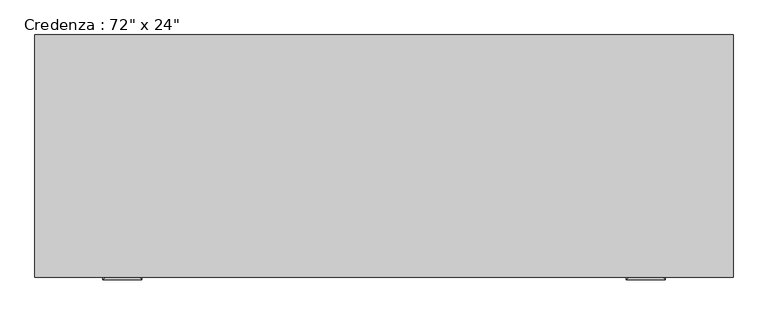
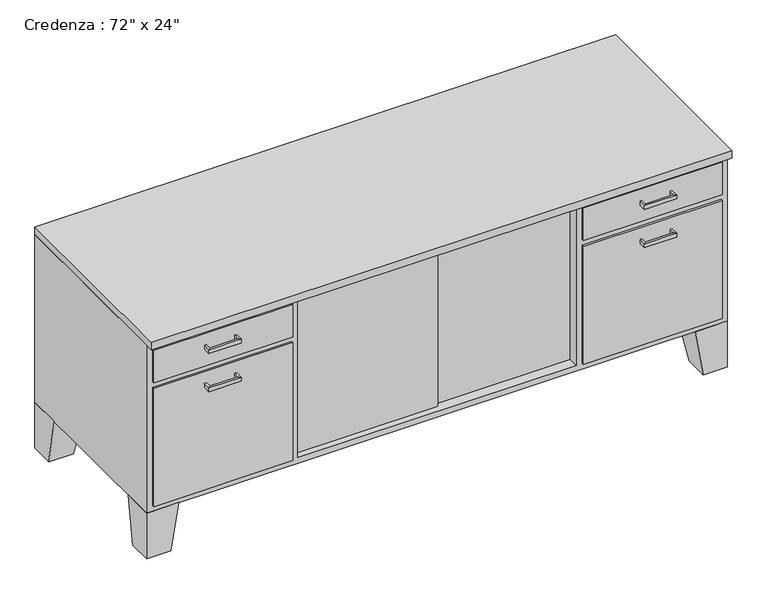
"""IFC4 building model written with IfcOpenShell, lengths in millimetres: furniture geometry."""

from ifc_helpers import new_model, si_unit, frame, origin, place, context, project, spatial, polyline, outline, extrude, faceted_brep, source, transform, mapped, element, save


def furniture_d4af3f8d(model_context):
    return source(origin(), model_context, "Body", "SolidModel", [
        extrude(outline(polyline([(531.7023176, -267.2714583), (46.8442623, -267.2714583), (46.8442623, -254.5714583), (531.7023176, -254.5714583), (531.7023176, -267.2714583)])), frame((0.0, 0.0, 171.45), z_axis=(0.0, 0.0, 1.0), x_axis=(1.0, 0.0, 0.0)), (0.0, 0.0, 1.0), 520.7),
        extrude(outline(polyline([(73.6254475, -279.9714583), (-378.6057377, -279.9714583), (-378.6057377, -267.2714583), (73.6254475, -267.2714583), (73.6254475, -279.9714583)])), frame((0.0, 0.0, 171.45), z_axis=(0.0, 0.0, 1.0), x_axis=(1.0, 0.0, 0.0)), (0.0, 0.0, 1.0), 520.7),
        faceted_brep([(872.3442623, 309.3803279, 152.4), (872.3442623, 207.7803279, 152.4), (973.9442623, 207.7803279, 152.4), (973.9442623, 309.3803279, 152.4), (897.7442623, 309.3803279, 0.0), (973.9442623, 309.3803279, 0.0), (973.9442623, 233.1803279, 0.0), (897.7442623, 233.1803279, 0.0)], [[[0, 1, 2, 3]], [[4, 5, 6, 7]], [[4, 7, 1, 0]], [[7, 6, 2, 1]], [[6, 5, 3, 2]], [[5, 4, 0, 3]]]),
        extrude(outline(polyline([(954.8942623, -306.5696721), (516.7442623, -306.5696721), (516.7442623, -300.2196721), (954.8942623, -300.2196721), (954.8942623, -306.5696721)])), frame((0.0, 0.0, 584.2), z_axis=(0.0, 0.0, 1.0), x_axis=(1.0, 0.0, 0.0)), (0.0, 0.0, 1.0), 107.95),
        extrude(outline(polyline([(954.8942623, -306.5696721), (516.7442623, -306.5696721), (516.7442623, -300.2196721), (954.8942623, -300.2196721), (954.8942623, -306.5696721)])), frame((0.0, 0.0, 171.45), z_axis=(0.0, 0.0, 1.0), x_axis=(1.0, 0.0, 0.0)), (0.0, 0.0, 1.0), 393.7),
        extrude(outline(polyline([(-397.6557377, -306.5696721), (-835.8057377, -306.5696721), (-835.8057377, -300.2196721), (-397.6557377, -300.2196721), (-397.6557377, -306.5696721)])), frame((0.0, 0.0, 584.2), z_axis=(0.0, 0.0, 1.0), x_axis=(1.0, 0.0, 0.0)), (0.0, 0.0, 1.0), 107.95),
        extrude(outline(polyline([(-397.6557377, -306.5696721), (-835.8057377, -306.5696721), (-835.8057377, -300.2196721), (-397.6557377, -300.2196721), (-397.6557377, -306.5696721)])), frame((0.0, 0.0, 171.45), z_axis=(0.0, 0.0, 1.0), x_axis=(1.0, 0.0, 0.0)), (0.0, 0.0, 1.0), 393.7),
        faceted_brep([(-753.2557377, -300.2196721, 152.4), (-753.2557377, -198.6196721, 152.4), (-854.8557377, -198.6196721, 152.4), (-854.8557377, -300.2196721, 152.4), (-778.6557377, -300.2196721, 0.0), (-854.8557377, -300.2196721, 0.0), (-854.8557377, -224.0196721, 0.0), (-778.6557377, -224.0196721, 0.0)], [[[0, 1, 2, 3]], [[4, 5, 6, 7]], [[4, 7, 1, 0]], [[7, 6, 2, 1]], [[6, 5, 3, 2]], [[5, 4, 0, 3]]]),
        faceted_brep([(-753.2557377, 309.3803279, 152.4), (-854.8557377, 309.3803279, 152.4), (-854.8557377, 207.7803279, 152.4), (-753.2557377, 207.7803279, 152.4), (-778.6557377, 309.3803279, 0.0), (-778.6557377, 233.1803279, 0.0), (-854.8557377, 233.1803279, 0.0), (-854.8557377, 309.3803279, 0.0)], [[[0, 1, 2, 3]], [[4, 5, 6, 7]], [[4, 7, 1, 0]], [[7, 6, 2, 1]], [[6, 5, 3, 2]], [[5, 4, 0, 3]]]),
        faceted_brep([(872.3442623, -300.2196721, 152.4), (973.9442623, -300.2196721, 152.4), (973.9442623, -198.6196721, 152.4), (872.3442623, -198.6196721, 152.4), (897.7442623, -300.2196721, 0.0), (897.7442623, -224.0196721, 0.0), (973.9442623, -224.0196721, 0.0), (973.9442623, -300.2196721, 0.0)], [[[0, 1, 2, 3]], [[4, 5, 6, 7]], [[4, 7, 1, 0]], [[7, 6, 2, 1]], [[6, 5, 3, 2]], [[5, 4, 0, 3]]]),
        faceted_brep([(973.9442623, 309.3803279, 711.2), (-854.8557377, 309.3803279, 711.2), (-854.8557377, -300.2196721, 711.2), (973.9442623, -300.2196721, 711.2), (973.9442623, 309.3803279, 152.4), (973.9442623, -300.2196721, 152.4), (-854.8557377, -300.2196721, 152.4), (-854.8557377, 309.3803279, 152.4), (-378.6057377, -300.2196721, 692.15), (497.6942623, -300.2196721, 692.15), (497.6942623, -300.2196721, 171.45), (-378.6057377, -300.2196721, 171.45), (497.6942623, 290.3303279, 692.15), (-378.6057377, 290.3303279, 692.15), (-378.6057377, 290.3303279, 171.45), (497.6942623, 290.3303279, 171.45)], [[[0, 1, 2, 3]], [[4, 5, 6, 7]], [[1, 0, 4, 7]], [[2, 1, 7, 6]], [[3, 2, 6, 5], [8, 9, 10, 11]], [[0, 3, 5, 4]], [[12, 13, 14, 15]], [[13, 12, 9, 8]], [[14, 13, 8, 11]], [[15, 14, 11, 10]], [[12, 15, 10, 9]]]),
        extrude(outline(polyline([(973.9442623, 309.3803279), (973.9442623, -325.6196721), (-854.8557377, -325.6196721), (-854.8557377, 309.3803279), (973.9442623, 309.3803279)])), frame((0.0, 0.0, 711.2), z_axis=(0.0, 0.0, 1.0), x_axis=(1.0, 0.0, 0.0)), (0.0, 0.0, 1.0), 25.4),
        faceted_brep([(-670.7057377, -306.5696721, 527.05), (-670.7057377, -306.5696721, 514.35), (-677.0557377, -306.5696721, 514.35), (-677.0557377, -306.5696721, 527.05), (-670.7057377, -325.6196721, 527.05), (-670.7057377, -325.6196721, 514.35), (-677.0557377, -331.9696721, 514.35), (-677.0557377, -331.9696721, 527.05), (-581.8057377, -325.6196721, 527.05), (-581.8057377, -325.6196721, 514.35), (-575.4557377, -331.9696721, 514.35), (-575.4557377, -331.9696721, 527.05), (-581.8057377, -306.5696721, 527.05), (-575.4557377, -306.5696721, 527.05), (-575.4557377, -306.5696721, 514.35), (-581.8057377, -306.5696721, 514.35)], [[[0, 1, 2, 3]], [[1, 0, 4, 5]], [[2, 1, 5, 6]], [[3, 2, 6, 7]], [[0, 3, 7, 4]], [[5, 4, 8, 9]], [[6, 5, 9, 10]], [[7, 6, 10, 11]], [[4, 7, 11, 8]], [[12, 13, 14, 15]], [[9, 8, 12, 15]], [[10, 9, 15, 14]], [[11, 10, 14, 13]], [[8, 11, 13, 12]]]),
        faceted_brep([(-670.7057377, -306.5696721, 654.05), (-670.7057377, -306.5696721, 641.35), (-677.0557377, -306.5696721, 641.35), (-677.0557377, -306.5696721, 654.05), (-670.7057377, -325.6196721, 654.05), (-670.7057377, -325.6196721, 641.35), (-677.0557377, -331.9696721, 641.35), (-677.0557377, -331.9696721, 654.05), (-581.8057377, -325.6196721, 654.05), (-581.8057377, -325.6196721, 641.35), (-575.4557377, -331.9696721, 641.35), (-575.4557377, -331.9696721, 654.05), (-581.8057377, -306.5696721, 654.05), (-575.4557377, -306.5696721, 654.05), (-575.4557377, -306.5696721, 641.35), (-581.8057377, -306.5696721, 641.35)], [[[0, 1, 2, 3]], [[1, 0, 4, 5]], [[2, 1, 5, 6]], [[3, 2, 6, 7]], [[0, 3, 7, 4]], [[5, 4, 8, 9]], [[6, 5, 9, 10]], [[7, 6, 10, 11]], [[4, 7, 11, 8]], [[12, 13, 14, 15]], [[9, 8, 12, 15]], [[10, 9, 15, 14]], [[11, 10, 14, 13]], [[8, 11, 13, 12]]]),
        faceted_brep([(700.8942623, -306.5696721, 654.1373112), (700.8942623, -306.5696721, 641.4373112), (694.5442623, -306.5696721, 641.4373112), (694.5442623, -306.5696721, 654.1373112), (700.8942623, -325.6196721, 654.1373112), (700.8942623, -325.6196721, 641.4373112), (694.5442623, -331.9696721, 641.4373112), (694.5442623, -331.9696721, 654.1373112), (789.7942623, -325.6196721, 654.1373112), (789.7942623, -325.6196721, 641.4373112), (796.1442623, -331.9696721, 641.4373112), (796.1442623, -331.9696721, 654.1373112), (789.7942623, -306.5696721, 654.1373112), (796.1442623, -306.5696721, 654.1373112), (796.1442623, -306.5696721, 641.4373112), (789.7942623, -306.5696721, 641.4373112)], [[[0, 1, 2, 3]], [[1, 0, 4, 5]], [[2, 1, 5, 6]], [[3, 2, 6, 7]], [[0, 3, 7, 4]], [[5, 4, 8, 9]], [[6, 5, 9, 10]], [[7, 6, 10, 11]], [[4, 7, 11, 8]], [[12, 13, 14, 15]], [[9, 8, 12, 15]], [[10, 9, 15, 14]], [[11, 10, 14, 13]], [[8, 11, 13, 12]]]),
        faceted_brep([(700.8942623, -306.5696721, 527.05), (700.8942623, -306.5696721, 514.35), (694.5442623, -306.5696721, 514.35), (694.5442623, -306.5696721, 527.05), (700.8942623, -325.6196721, 527.05), (700.8942623, -325.6196721, 514.35), (694.5442623, -331.9696721, 514.35), (694.5442623, -331.9696721, 527.05), (789.7942623, -325.6196721, 527.05), (789.7942623, -325.6196721, 514.35), (796.1442623, -331.9696721, 514.35), (796.1442623, -331.9696721, 527.05), (789.7942623, -306.5696721, 527.05), (796.1442623, -306.5696721, 527.05), (796.1442623, -306.5696721, 514.35), (789.7942623, -306.5696721, 514.35)], [[[0, 1, 2, 3]], [[1, 0, 4, 5]], [[2, 1, 5, 6]], [[3, 2, 6, 7]], [[0, 3, 7, 4]], [[5, 4, 8, 9]], [[6, 5, 9, 10]], [[7, 6, 10, 11]], [[4, 7, 11, 8]], [[12, 13, 14, 15]], [[9, 8, 12, 15]], [[10, 9, 15, 14]], [[11, 10, 14, 13]], [[8, 11, 13, 12]]]),
    ])


if __name__ == "__main__":
    model = new_model("IFC4")
    model_context = context("Model", 3, world=origin())
    ifc_project = project(units=[si_unit("LENGTHUNIT", "METRE", prefix="MILLI")], contexts=[model_context])
    site = spatial("IfcSite", under=ifc_project)
    building = spatial("IfcBuilding", under=site)
    placement = place(None, origin())
    furniture_shape = furniture_d4af3f8d(model_context)
    element("IfcFurniture", 1, ObjectType="Credenza : 72\" x 24\"", at=placement, inside=building, context=model_context, shape_type="MappedRepresentation", body=[
        mapped(furniture_shape, transform((0.0, 0.0, 0.0), x_axis=(1.0, 0.0, 0.0), y_axis=(0.0, 1.0, 0.0), z_axis=(0.0, 0.0, 1.0))),
    ])
    save(model, "model.ifc")

# Revit data of these elements
# Type "Credenza : 72\" x 24\""
#   Assembly Code = "E2020200"
#   Depth = 2' - 0"
#   Height = 2' - 5"
#   Width = 6' - 0"
#   Body Material = Laminate, Ivory, Matte
#   Handles/Legs Material = Steel, Chrome Plated
#   Top Material = Cherry
#   Default Elevation = 0
# Element 1 (IfcFurniture, "Credenza : 72\" x 24\"")
#   Materials on its faces: "Steel, Chrome Plated", "Laminate, Ivory, Matte", "Cherry"
# Materials
#   "Laminate, Ivory, Matte": class "Plastic", colour RGB 247 247 239, transparency 0, Description = "Plastic Laminate - Ivory, Matte", Cost = 0
#   "Steel, Chrome Plated": class "Metal", colour RGB 17 17 17, transparency 0, Description = "Chromiuim plated steel", Cost = 0
#   "Cherry": class "Wood", colour RGB 226 177 128, transparency 0, Description = "Prunus Serotina", Cost = 0
